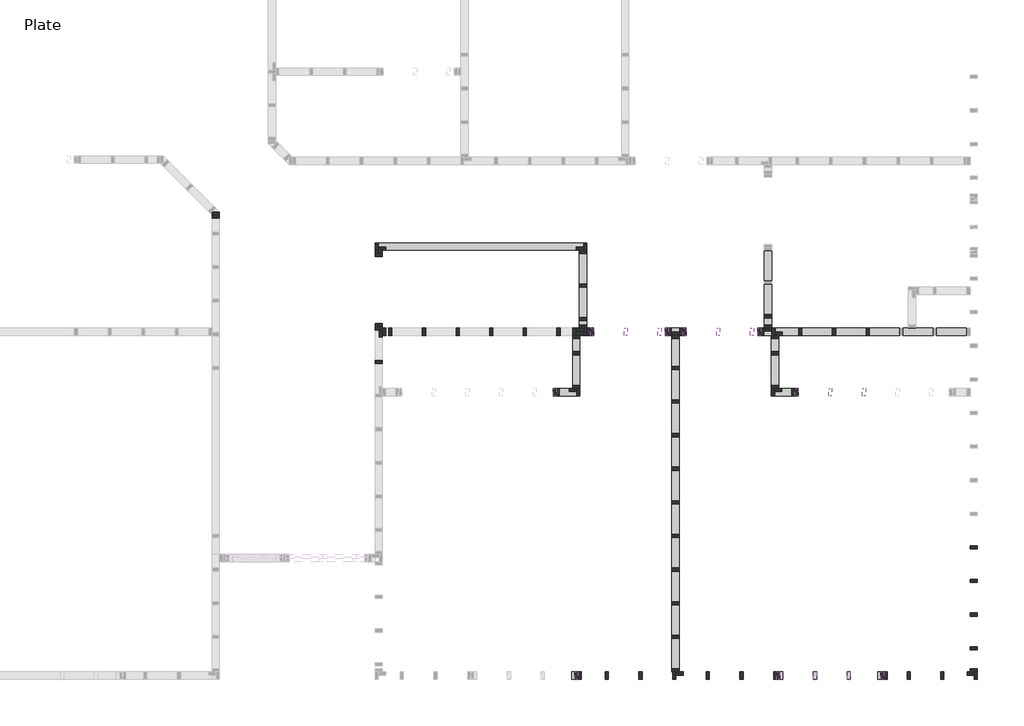
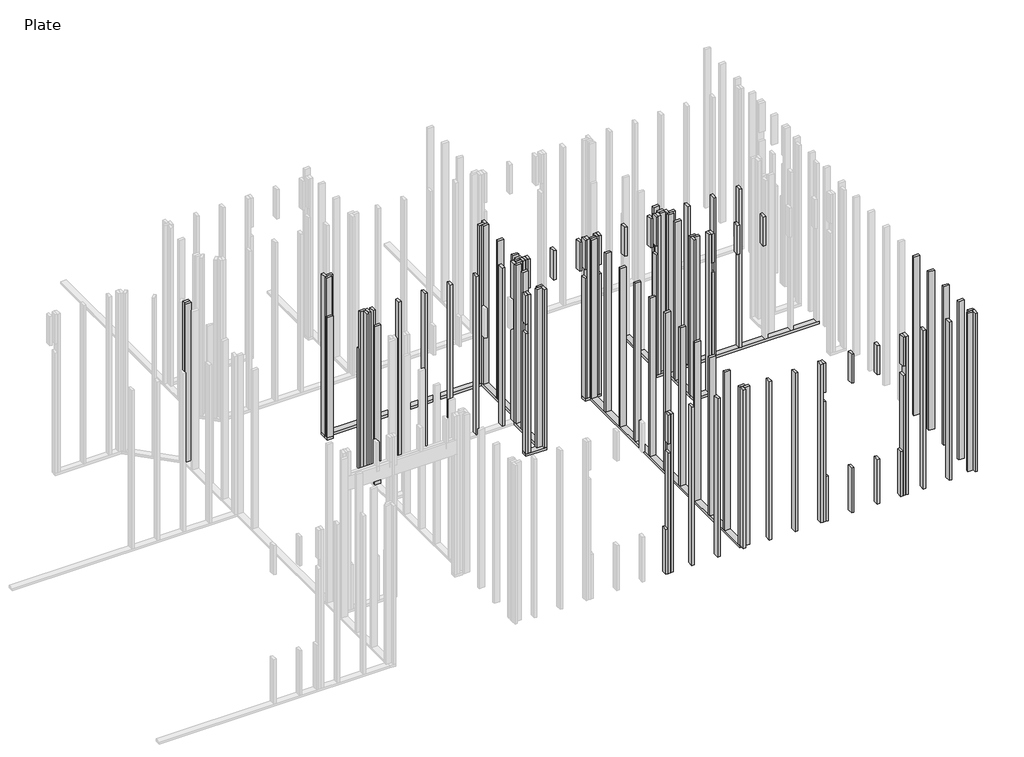
# One storey, part 2 of 5: 112 columns, 11 beams.
# Revit data of these elements (continued)
# Type "Dimension Lumber : Supporting Bottom Plate"
#   Assembly Code = "B10"
#   A = 0.0364583 SF
#   Length [instance default] = 5' - 0"
#   b = 0' - 3 1/2"
#   d = 0' - 1 1/2"
#   Structural Material [instance default] = Softwood, Lumber
# Type "Dimension Lumber-Column : 2x4"
#   Int Type = "Interior"
#   Assembly Code = "B10"
#   Cost = 8.05
#   A = 0.0364583 SF
#   b = 0' - 1 1/2"
#   d = 0' - 3 1/2"
#   Structural Material [instance default] = Softwood, Lumber
# Elements 1, 3 (IfcBeam, "Dimension Lumber : Supporting Bottom Plate")
#   Comments = ""
#   Structural Material = Douglas Fir #2
#   Phase Created = New Construction
#   Materials on its faces: "Douglas Fir #2"
# Elements 2, 4, 5, 6, 7, 8, 9, 10, 11 (IfcBeam, "Dimension Lumber : Supporting Bottom Plate")
#   Structural Material = Douglas Fir #2
#   Phase Created = New Construction
#   Materials on its faces: "Douglas Fir #2"
# Elements 12, 13, 14, 15, 16, 17, 18, 19, 20, 21, 36, 37, 66, 67, 68, 69, 70, 71, 72, 91, 92, 93, 102, 103, 104, 105, 106 (IfcColumn, "Dimension Lumber-Column : 2x4")
#   Function = "Exterior"
#   Structural Material = Douglas Fir #2
#   Phase Created = New Construction
#   Materials on its faces: "Douglas Fir #2"
# Elements 22, 23, 24, 25, 26, 27, 28, 29, 30, 31, 32, 33, 34, 35, 38, 39, 40, 41, 42, 43, 44, 45, 46, 47, 48, 49, 50, 51, 52, 53, 54, 55, 56, 57, 58, 59, 60, 61, 62, 63, 64, 65, 73, 74, 75, 76, 77, 78, 79, 80, 81, 82, 83, 84, 85, 86, 87, 88, 89, 90, 94, 95, 96, 97, 98, 99, 100, 101, 107, 108, 109, 110, 111, 112, 113, 114, 115, 116, 117, 118 (IfcColumn, "Dimension Lumber-Column : 2x4")
#   Function = "Interior"
#   Structural Material = Douglas Fir #2
#   Phase Created = New Construction
#   Materials on its faces: "Douglas Fir #2"
# Elements 119, 120, 121, 122, 123 (IfcColumn, "Dimension Lumber-Column : 2x4")
#   Structural Material = Douglas Fir #2
#   Phase Created = New Construction
#   Materials on its faces: "Douglas Fir #2"
# Materials
#   "Softwood, Lumber": class "Wood", colour RGB 223 192 134, transparency 0, Description = "Pinus Echinata", Cost = 0
#   "Douglas Fir #2": class "Wood", colour RGB 223 192 134, transparency 0, Description = "Pinus Echinata", Cost = 0
